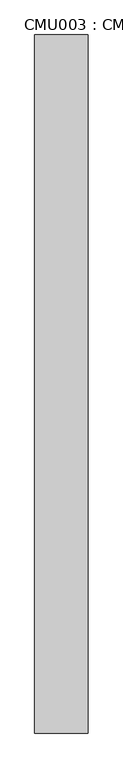
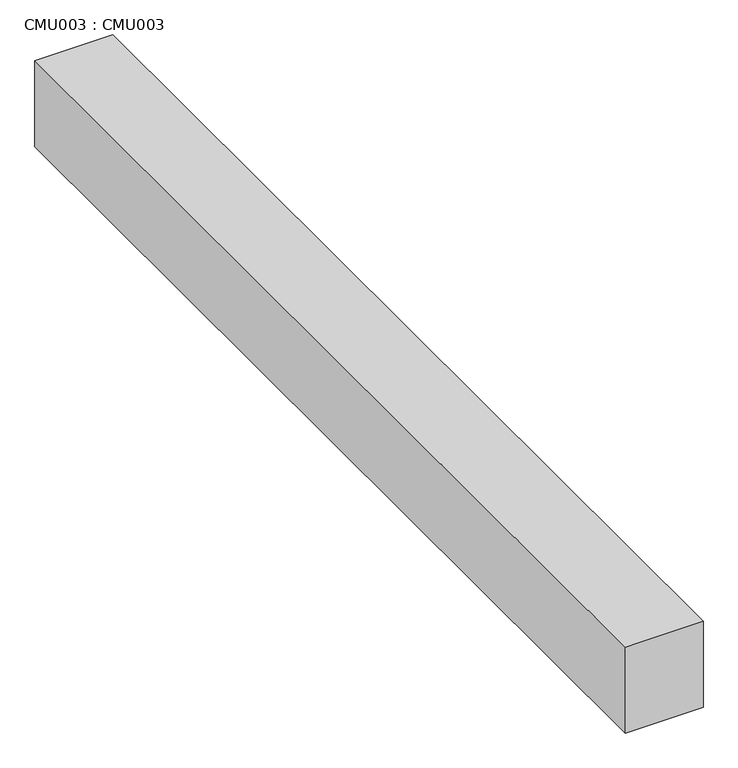
"""IFC4 building model written with IfcOpenShell, lengths in millimetres: proxy geometry, CMU003 : CMU003."""

from ifc_helpers import new_model, si_unit, frame, origin, place, context, project, spatial, polyline, outline, extrude, source, transform, mapped, element, save


def cmu003_cmu003_98a6b7b9(model_context):
    return source(origin(), model_context, "Body", "SweptSolid", [
        extrude(outline(polyline([(-10098.4737014, 7982.1531721), (-10250.8737014, 7982.1531721), (-10250.8737014, 9982.1531721), (-10098.4737014, 9982.1531721), (-10098.4737014, 7982.1531721)])), frame((0.0, 0.0, 33007.6325216), z_axis=(0.0, 0.0, 1.0), x_axis=(1.0, 0.0, 0.0)), (0.0, 0.0, 1.0), 177.8),
    ])


if __name__ == "__main__":
    model = new_model("IFC4")
    model_context = context("Model", 3, world=origin())
    ifc_project = project(units=[si_unit("LENGTHUNIT", "METRE", prefix="MILLI")], contexts=[model_context])
    site = spatial("IfcSite", under=ifc_project)
    building = spatial("IfcBuilding", under=site)
    placement = place(None, origin())
    cmu003_cmu003_shape = cmu003_cmu003_98a6b7b9(model_context)
    element("IfcBuildingElementProxy", 1, Name="CMU003 : CMU003", ObjectType="CMU003 : CMU003", at=placement, inside=building, context=model_context, shape_type="MappedRepresentation", body=[
        mapped(cmu003_cmu003_shape, transform((0.0, 0.0, 0.0), x_axis=(1.0, 0.0, 0.0), y_axis=(0.0, 1.0, 0.0), z_axis=(0.0, 0.0, 1.0))),
    ])
    save(model, "model.ifc")

# Revit data of these elements
# Type "CMU003 : CMU003"
#   NameOverride = "CMU003"
# Element 1 (IfcBuildingElementProxy, "CMU003 : CMU003")
#   Materials on its faces: "4\" CMU WALL"
# Materials
#   "4\" CMU WALL": class "Unassigned", colour RGB 128 128 128, transparency 0, Cost = 0
